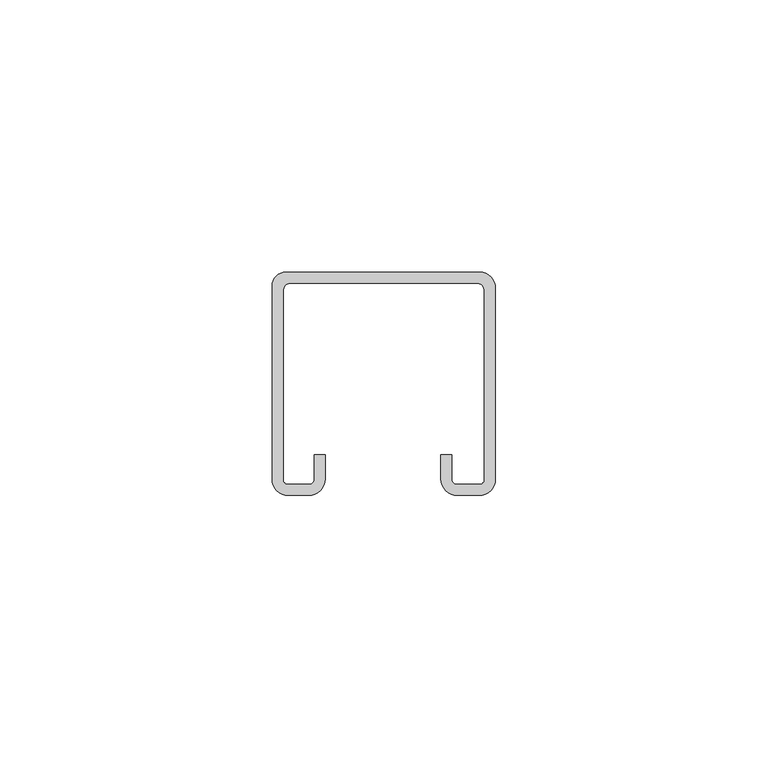
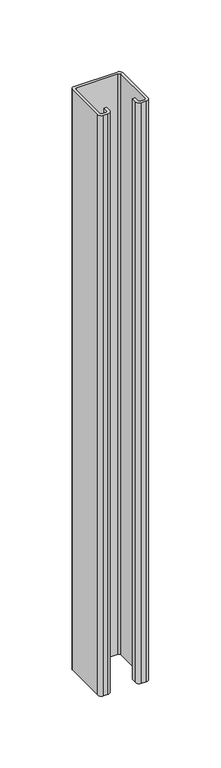
"""IFC4 building model written with IfcOpenShell, lengths in millimetres: proxy geometry, TN_Профиль монтажный : Профиль монтажный 41х41x2,0-3000."""

import ifcopenshell
import ifcopenshell.guid

model = None  # the IFC model being written
_history = None  # IfcOwnerHistory: only IFC2X3 demands one
_inside = {}  # id of a spatial element -> (the spatial element, [elements in it])
_under = {}  # id of a project, library or spatial element -> (it, [spatial elements below it])
_declared = {}  # id of a project -> (the project, [libraries it declares])
_typed = {}  # id of a type object -> (the type object, [elements of that type])
_made_of = {}  # id of a material, layer set ... -> (it, [elements and type objects made of it])


def new_model(schema):
    """Start an empty IFC model of exactly this schema.

    Asked for "IFC4X3", IfcOpenShell would pick the latest addendum, in which some entities
    have other attributes; the version numbers below select the first issue.
    IFC2X3 requires an IfcOwnerHistory on every rooted entity: one is made here for all.
    """
    global model, _history
    if schema == "IFC4X3":
        model = ifcopenshell.file(schema_version=(4, 3, 0, 0))
    else:
        model = ifcopenshell.file(schema=schema)
    _inside.clear()
    _under.clear()
    _declared.clear()
    _typed.clear()
    _made_of.clear()
    _history = None
    if model.schema == "IFC2X3":
        org = make("IfcOrganization", Name="unknown")
        user = make(
            "IfcPersonAndOrganization",
            ThePerson=make("IfcPerson", FamilyName="unknown"),
            TheOrganization=org,
        )
        app = make(
            "IfcApplication",
            ApplicationDeveloper=org,
            Version="unknown",
            ApplicationFullName="unknown",
            ApplicationIdentifier="unknown",
        )
        _history = make(
            "IfcOwnerHistory",
            OwningUser=user,
            OwningApplication=app,
            ChangeAction="ADDED",
            CreationDate=0,
        )
    return model


def make(cls, **values):
    """One entity of the class cls with the attributes given. An attribute that is None is left unset."""
    return model.create_entity(
        cls, **{name: value for name, value in values.items() if value is not None}
    )


def rooted(cls, **values):
    """An entity with a GlobalId (a new one), such as an element, a storey or a relation."""
    return make(cls, GlobalId=ifcopenshell.guid.new(), OwnerHistory=_history, **values)


def si_unit(unit_type, name, prefix=None):
    """IfcSIUnit, for example si_unit("LENGTHUNIT", "METRE", prefix="MILLI")."""
    return make("IfcSIUnit", UnitType=unit_type, Prefix=prefix, Name=name)


def assignment(units):
    """IfcUnitAssignment: the units of a project."""
    return None if units is None else make("IfcUnitAssignment", Units=units)


def point(xyz):
    """IfcCartesianPoint."""
    return None if xyz is None else make("IfcCartesianPoint", Coordinates=xyz)


def direction(xyz):
    """IfcDirection."""
    return None if xyz is None else make("IfcDirection", DirectionRatios=xyz)


def frame(location, z_axis=None, x_axis=None):
    """IfcAxis2Placement3D, a coordinate frame: its origin and axes. An axis left out is left unset."""
    return make(
        "IfcAxis2Placement3D",
        Location=point(location),
        Axis=direction(z_axis),
        RefDirection=direction(x_axis),
    )


def frame_2d(location, x_axis=None):
    """IfcAxis2Placement2D, a coordinate frame in the plane: its origin and x axis."""
    return make(
        "IfcAxis2Placement2D", Location=point(location), RefDirection=direction(x_axis)
    )


def origin():
    """The frame at (0, 0, 0) with its axes left unset."""
    return frame((0.0, 0.0, 0.0))


def origin_with_axes():
    """The frame at (0, 0, 0) with the z axis (0, 0, 1) and the x axis (1, 0, 0) written out."""
    return frame((0.0, 0.0, 0.0), z_axis=(0.0, 0.0, 1.0), x_axis=(1.0, 0.0, 0.0))


def place(relative_to, where):
    """IfcLocalPlacement: puts the frame where relative to a parent placement (None: the world)."""
    return make(
        "IfcLocalPlacement", PlacementRelTo=relative_to, RelativePlacement=where
    )


def context(
    kind, dimensions, precision=None, world=None, true_north=None, identifier=None
):
    """IfcGeometricRepresentationContext, for example the 3D "Model" context."""
    return make(
        "IfcGeometricRepresentationContext",
        ContextIdentifier=identifier,
        ContextType=kind,
        CoordinateSpaceDimension=dimensions,
        Precision=precision,
        WorldCoordinateSystem=world,
        TrueNorth=true_north,
    )


def project(units=None, contexts=None):
    """IfcProject with its units and contexts."""
    return rooted(
        "IfcProject",
        Name="project",
        RepresentationContexts=contexts,
        UnitsInContext=assignment(units),
    )


def spatial(cls, under=None, at=None, **own):
    """A site, building, storey or space (cls), placed at a placement, below another one or the project."""
    s = rooted(cls, ObjectPlacement=at, **own)
    if under is not None:
        _under.setdefault(under.id(), (under, []))[1].append(s)
    return s


def polyline(points):
    """IfcPolyline through the points."""
    return make("IfcPolyline", Points=[point(p) for p in points])


def circle_curve(where, radius):
    """IfcCircle in the frame where."""
    return make("IfcCircle", Position=where, Radius=radius)


def trimmed(basis, trim1, trim2, sense, master):
    """IfcTrimmedCurve: the piece of a basis curve between two trims."""
    return make(
        "IfcTrimmedCurve",
        BasisCurve=basis,
        Trim1=trim1,
        Trim2=trim2,
        SenseAgreement=sense,
        MasterRepresentation=master,
    )


def segment(curve, same_sense, transition):
    """IfcCompositeCurveSegment."""
    return make(
        "IfcCompositeCurveSegment",
        Transition=transition,
        SameSense=same_sense,
        ParentCurve=curve,
    )


def composite_curve(segments, self_intersect=None):
    """IfcCompositeCurve: segments joined end to end."""
    return make("IfcCompositeCurve", Segments=segments, SelfIntersect=self_intersect)


def outline(outer, holes=None, kind="AREA"):
    """IfcArbitraryClosedProfileDef: a profile drawn as a closed curve; with holes, ...WithVoids."""
    if holes is None:
        return make("IfcArbitraryClosedProfileDef", ProfileType=kind, OuterCurve=outer)
    return make(
        "IfcArbitraryProfileDefWithVoids",
        ProfileType=kind,
        OuterCurve=outer,
        InnerCurves=holes,
    )


def extrude(swept, where, along, depth):
    """IfcExtrudedAreaSolid: the profile swept, set in the frame where, extruded along a direction by depth."""
    return make(
        "IfcExtrudedAreaSolid",
        SweptArea=swept,
        Position=where,
        ExtrudedDirection=direction(along),
        Depth=depth,
    )


def shape(context_of_items, identifier, shape_type, items):
    """IfcShapeRepresentation: the items that make up one representation, for example the "Body"."""
    return make(
        "IfcShapeRepresentation",
        ContextOfItems=context_of_items,
        RepresentationIdentifier=identifier,
        RepresentationType=shape_type,
        Items=items,
    )


def source(mapping_origin, context_of_items, identifier, shape_type, items):
    """IfcRepresentationMap: a shape defined once, which mapped items show again and again."""
    return make(
        "IfcRepresentationMap",
        MappingOrigin=mapping_origin,
        MappedRepresentation=shape(context_of_items, identifier, shape_type, items),
    )


def transform(
    local_origin,
    x_axis=None,
    y_axis=None,
    z_axis=None,
    scale=None,
    scale2=None,
    scale3=None,
    uniform=True,
):
    """IfcCartesianTransformationOperator3D, or its non-uniform kind. x_axis, y_axis, z_axis: its Axis1, 2, 3."""
    if uniform:
        return make(
            "IfcCartesianTransformationOperator3D",
            Axis1=direction(x_axis),
            Axis2=direction(y_axis),
            LocalOrigin=point(local_origin),
            Scale=scale,
            Axis3=direction(z_axis),
        )
    return make(
        "IfcCartesianTransformationOperator3DnonUniform",
        Axis1=direction(x_axis),
        Axis2=direction(y_axis),
        LocalOrigin=point(local_origin),
        Scale=scale,
        Axis3=direction(z_axis),
        Scale2=scale2,
        Scale3=scale3,
    )


def mapped(mapping_source, mapping_target):
    """IfcMappedItem: shows the shape of a source again, moved by a transform."""
    return make(
        "IfcMappedItem", MappingSource=mapping_source, MappingTarget=mapping_target
    )


def made_of(thing, what):
    """Note that an element or type object is made of a material, layer set ...; save() writes the relation."""
    if what is not None:
        _made_of.setdefault(what.id(), (what, []))[1].append(thing)
    return thing


def element(
    cls,
    number,
    at=None,
    inside=None,
    cuts=None,
    type_object=None,
    material=None,
    context=None,
    identifier="Body",
    shape_type=None,
    held_by="IfcProductDefinitionShape",
    body=None,
    shapes=None,
    **own,
):
    """One element of the class cls, such as IfcWall. Its Tag is "e" and its number.

    at: its placement. inside: the storey or other place that contains it. cuts: it is an
    opening in that element (IfcRelVoidsElement). A single representation is given by context,
    identifier, shape_type and body (its items); several are given by shapes. held_by: the class
    of the entity that holds the representations. save() writes the other relations.
    """
    e = rooted(cls, Tag="e%d" % number, ObjectPlacement=at, **own)
    if body is not None:
        shapes = [shape(context, identifier, shape_type, body)]
    if shapes is not None:
        e.Representation = make(held_by, Representations=shapes)
    if inside is not None:
        _inside.setdefault(inside.id(), (inside, []))[1].append(e)
    if cuts is not None:
        rooted(
            "IfcRelVoidsElement", RelatingBuildingElement=cuts, RelatedOpeningElement=e
        )
    if type_object is not None:
        _typed.setdefault(type_object.id(), (type_object, []))[1].append(e)
    return made_of(e, material)


def aggregate(whole, parts):
    """IfcRelAggregates: a whole, such as a stair, and the parts it consists of."""
    return rooted("IfcRelAggregates", RelatingObject=whole, RelatedObjects=parts)


def save(model, path):
    """Write the relations noted so far, then the file.

    IfcRelAggregates (storeys below a building ...), IfcRelContainedInSpatialStructure (elements
    in a storey), IfcRelDefinesByType, IfcRelAssociatesMaterial and IfcRelDeclares: one each for
    every whole, place, type object, material and project.
    """
    for whole, parts in _under.values():
        aggregate(whole, parts)
    for where, things in _inside.values():
        rooted(
            "IfcRelContainedInSpatialStructure",
            RelatedElements=things,
            RelatingStructure=where,
        )
    for kind, things in _typed.values():
        rooted("IfcRelDefinesByType", RelatedObjects=things, RelatingType=kind)
    for what, things in _made_of.values():
        rooted("IfcRelAssociatesMaterial", RelatedObjects=things, RelatingMaterial=what)
    for by, libraries in _declared.values():
        rooted("IfcRelDeclares", RelatingContext=by, RelatedDefinitions=libraries)
    model.write(path)


def generic_models_7f36e49c(model_context):
    return source(origin(), model_context, "Body", "SweptSolid", [
        extrude(outline(composite_curve([segment(polyline([(20.7157599, -2.9315199), (20.7157599, -38.0)]), True, "CONTINUOUS"), segment(trimmed(circle_curve(frame_2d((17.7157599, -38.0)), 3.0), [point((20.7157599, -38.0))], [point((17.7157599, -41.0))], False, "CARTESIAN"), True, "CONTINUOUS"), segment(polyline([(17.7157599, -41.0), (13.7568638, -41.0)]), True, "CONTINUOUS"), segment(trimmed(circle_curve(frame_2d((13.7568638, -37.9588961)), 3.0411039), [point((13.7568638, -41.0))], [point((10.7157599, -37.9588961))], False, "CARTESIAN"), True, "CONTINUOUS"), segment(polyline([(10.7157599, -37.9588961), (10.7157599, -33.5), (12.7157599, -33.5), (12.7157599, -38.0)]), True, "CONTINUOUS"), segment(trimmed(circle_curve(frame_2d((13.7157599, -38.0)), 1.0), [point((12.7157599, -38.0))], [point((13.7157599, -39.0))], True, "CARTESIAN"), True, "CONTINUOUS"), segment(polyline([(13.7157599, -39.0), (17.7157599, -39.0)]), True, "CONTINUOUS"), segment(trimmed(circle_curve(frame_2d((17.7157599, -38.0)), 1.0), [point((17.7157599, -39.0))], [point((18.7157599, -38.0))], True, "CARTESIAN"), True, "CONTINUOUS"), segment(polyline([(18.7157599, -38.0), (18.7157599, -3.5)]), True, "CONTINUOUS"), segment(trimmed(circle_curve(frame_2d((17.2157599, -3.5)), 1.5), [point((18.7157599, -3.5))], [point((17.2157599, -2.0))], True, "CARTESIAN"), True, "CONTINUOUS"), segment(polyline([(17.2157599, -2.0), (-16.7842401, -2.0)]), True, "CONTINUOUS"), segment(trimmed(circle_curve(frame_2d((-16.7842401, -3.5)), 1.5), [point((-16.7842401, -2.0))], [point((-18.2842401, -3.5))], True, "CARTESIAN"), True, "CONTINUOUS"), segment(polyline([(-18.2842401, -3.5), (-18.2842401, -38.0)]), True, "CONTINUOUS"), segment(trimmed(circle_curve(frame_2d((-17.2842401, -38.0)), 1.0), [point((-18.2842401, -38.0))], [point((-17.2842401, -39.0))], True, "CARTESIAN"), True, "CONTINUOUS"), segment(polyline([(-17.2842401, -39.0), (-13.5684801, -39.0)]), True, "CONTINUOUS"), segment(trimmed(circle_curve(frame_2d((-13.5684801, -38.0)), 1.0), [point((-13.5684801, -39.0))], [point((-12.5684801, -38.0))], True, "CARTESIAN"), True, "CONTINUOUS"), segment(polyline([(-12.5684801, -38.0), (-12.5684801, -33.5), (-10.5684801, -33.5), (-10.5684801, -38.0)]), True, "CONTINUOUS"), segment(trimmed(circle_curve(frame_2d((-13.5684801, -38.0)), 3.0), [point((-10.5684801, -38.0))], [point((-13.5684801, -41.0))], False, "CARTESIAN"), True, "CONTINUOUS"), segment(polyline([(-13.5684801, -41.0), (-17.2842401, -41.0)]), True, "CONTINUOUS"), segment(trimmed(circle_curve(frame_2d((-17.2842401, -38.0)), 3.0), [point((-17.2842401, -41.0))], [point((-20.2842401, -38.0))], False, "CARTESIAN"), True, "CONTINUOUS"), segment(polyline([(-20.2842401, -38.0), (-20.2842401, -2.5)]), True, "CONTINUOUS"), segment(trimmed(circle_curve(frame_2d((-17.7842401, -2.5)), 2.5), [point((-20.2842401, -2.5))], [point((-17.7842401, 0.0))], False, "CARTESIAN"), True, "CONTINUOUS"), segment(polyline([(-17.7842401, 0.0), (17.7842401, 0.0)]), True, "CONTINUOUS"), segment(trimmed(circle_curve(frame_2d((17.7842401, -2.9315199)), 2.9315199), [point((17.7842401, 0.0))], [point((20.7157599, -2.9315199))], False, "CARTESIAN"), True, "CONTINUOUS")], self_intersect=False)), origin_with_axes(), (0.0, 0.0, 1.0), 500.0),
    ])


if __name__ == "__main__":
    model = new_model("IFC4")
    model_context = context("Model", 3, world=origin())
    ifc_project = project(units=[si_unit("LENGTHUNIT", "METRE", prefix="MILLI")], contexts=[model_context])
    site = spatial("IfcSite", under=ifc_project)
    building = spatial("IfcBuilding", under=site)
    placement = place(None, origin())
    generic_models_shape = generic_models_7f36e49c(model_context)
    element("IfcBuildingElementProxy", 1, Name="TN_Профиль монтажный : Профиль монтажный 41х41x2,0-3000", ObjectType="TN_Профиль монтажный : Профиль монтажный 41х41x2,0-3000", at=placement, inside=building, context=model_context, shape_type="MappedRepresentation", body=[
        mapped(generic_models_shape, transform((0.0, 0.0, 0.0), x_axis=(1.0, 0.0, 0.0), y_axis=(0.0, 1.0, 0.0), z_axis=(0.0, 0.0, 1.0))),
    ])
    save(model, "model.ifc")

# Revit data of these elements
# Type "TN_Профиль монтажный : Профиль монтажный 41х41x2,0-3000"
#   Description = "Профиль монтажный – траверса С-образной формы предназначен для горизонтального и вертикального монтажа тяжелых инженерных систем, оборудования систем вентиляции и кондиционирования, установок электроснабжения, элементов трубопроводов, также для изготовления стенных консолей пристенного монтажа, рам оснований различного типа под оборудование. Возможно замещение на основе сконструированных модулей серийных опор ГОСТ для раскрепления технологических трубопроводов. Рекомендуется для применения в сухих, влажных помещениях и на открытом воздухе."
#   Manufacturer = "ТехноНИКОЛЬ"
#   Model = "Комплектующие к опорам"
#   URL = "https://nav.tn.ru/knowledge-base/polimernye-membrany/opory-pod-oborudovanie-na-ploskoy-krovle/?sphrase_id=266812"
#   ADSK_Обозначение = "ТехноНИКОЛЬ"
#   ADSK_Наименование краткое = "П41х41x2,0"
#   ADSK_Наименование = "Профиль монтажный 41х41x2,0-3000"
#   ADSK_Масса_Текст = ""
#   ADSK_Марка = "П41х41x2,0"
#   ADSK_Код изделия = "660816"
#   ADSK_Завод-изготовитель = "ТехноНИКОЛЬ"
#   ADSK_Единица измерения = "п.м."
#   ADSK_Группирование = "Комплектующие к опорам"
#   ADSK_URL страницы изделия = "https://nav.tn.ru/knowledge-base/polimernye-membrany/opory-pod-oborudovanie-na-ploskoy-krovle/?sphrase_id=266812"
#   ADSK_URL документации изделия = ""
#   Размер_Длина_Вводимая [instance default] = 1000 mm
#   ADSK_Размер_Длина [instance default] = 1000 mm
#   ADSK_Количество [instance default] = 1
#   Тип профиля = 1
#   Профиль монтажный 41х41x2,0 = yes
#   Профиль монтажный 41x62x2,5 = no
#   Профиль монтажный 41x124x2,5 = no
#   ADSK_Материал = TN_СтальГальванизированная_Серый
#   Default Elevation = 0
# Element 1 (IfcBuildingElementProxy, "TN_Профиль монтажный : Профиль монтажный 41х41x2,0-3000")
#   Размер_Длина_Вводимая = 500 mm
#   ADSK_Размер_Длина = 500 mm
#   ADSK_Количество = 0.5
#   Materials on its faces: "TN_СтальГальванизированная_Серый"
# Materials
#   "TN_СтальГальванизированная_Серый": class "Типовые", colour RGB 206 210 213, transparency 0, Cost = 0
